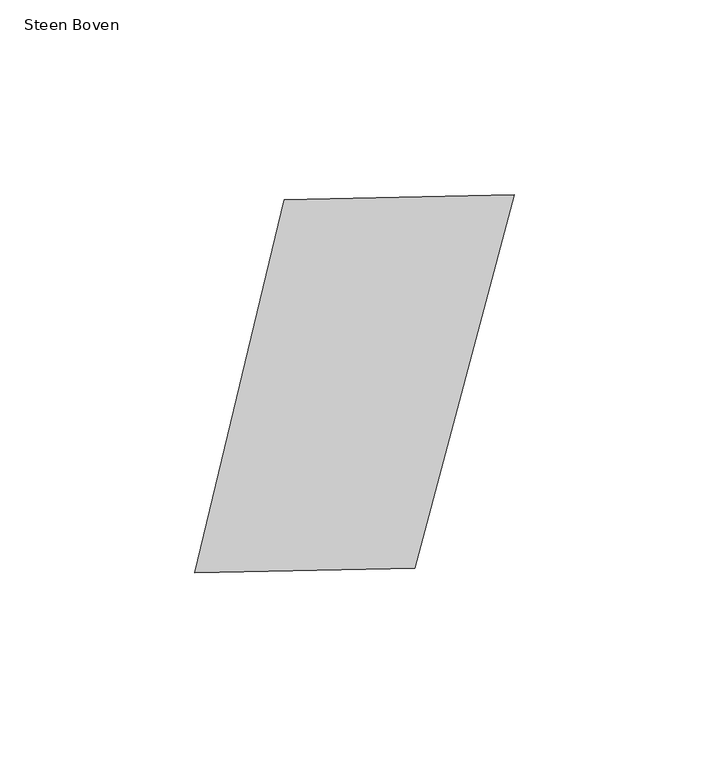
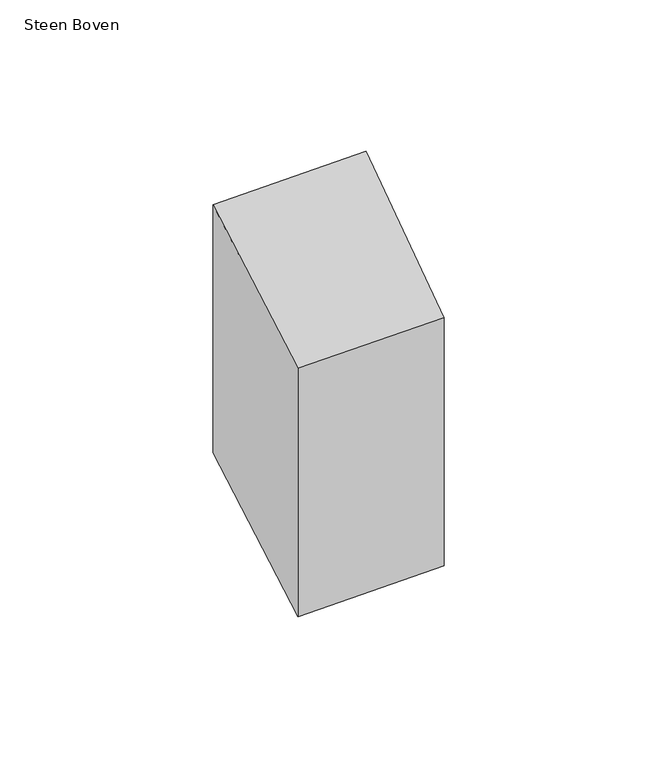
"""IFC4 building model written with IfcOpenShell, lengths in millimetres: proxy geometry, 00_GMA_steen_versie_4 : Steen Boven."""

from ifc_helpers import new_model, si_unit, origin, origin_with_axes, place, context, project, spatial, polyline, outline, extrude, source, transform, mapped, element, save


def steen_boven_9cbfec4d(model_context):
    return source(origin(), model_context, "Body", "SweptSolid", [
        extrude(outline(polyline([(113.9568566, 118.7889283), (88.4390091, 23.0223042), (32.1209988, 21.8380681), (55.0050159, 117.5190081), (113.9568566, 118.7889283)])), origin_with_axes(), (0.0, 0.0, 1.0), 100.0),
    ])


if __name__ == "__main__":
    model = new_model("IFC4")
    model_context = context("Model", 3, world=origin())
    ifc_project = project(units=[si_unit("LENGTHUNIT", "METRE", prefix="MILLI")], contexts=[model_context])
    site = spatial("IfcSite", under=ifc_project)
    building = spatial("IfcBuilding", under=site)
    placement = place(None, origin())
    steen_boven_shape = steen_boven_9cbfec4d(model_context)
    element("IfcBuildingElementProxy", 1, Name="00_GMA_steen_versie_4 : Steen Boven", ObjectType="00_GMA_steen_versie_4 : Steen Boven", at=placement, inside=building, context=model_context, shape_type="MappedRepresentation", body=[
        mapped(steen_boven_shape, transform((0.0, 0.0, 0.0), x_axis=(1.0, 0.0, 0.0), y_axis=(0.0, 1.0, 0.0), z_axis=(0.0, 0.0, 1.0))),
    ])
    save(model, "model.ifc")

# Revit data of these elements
# Type "00_GMA_steen_versie_4 : Steen Boven"
#   StootVoegHalfBoven [instance default] = 5 mm
#   StootVoegHalf [instance default] = 5 mm
#   StootVoegBreedteOnder = 10 mm
#   StootVoegBreedteBoven = 10 mm
#   Steendikte = 100 mm
#   LintVoegOnderHalf = 5 mm
#   LintVoegOnder = 10 mm
#   LintVoegBovenHalf = 0 mm
#   LintVoegBoven = 0 mm
#   materiaal = none
#   MateriaalVoeg = none
#   Default Elevation = 0
